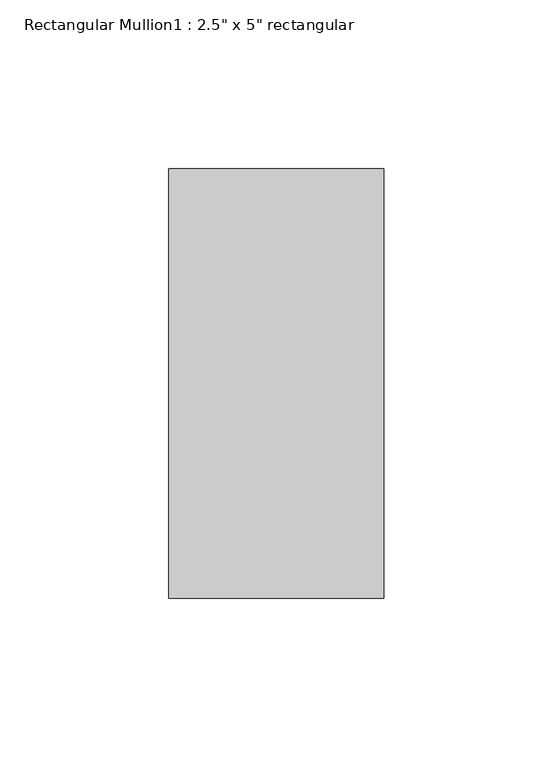
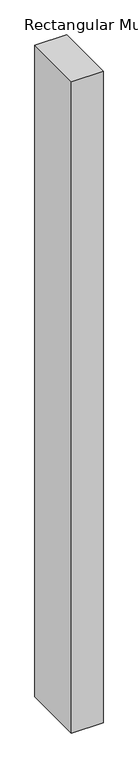
"""IFC4 building model written with IfcOpenShell, lengths in millimetres: member geometry."""

from ifc_helpers import new_model, si_unit, frame, origin, place, context, project, spatial, polyline, outline, extrude, source, transform, mapped, element, save


def member_8caa64b4(model_context):
    return source(origin(), model_context, "Body", "SweptSolid", [
        extrude(outline(polyline([(31.75, 63.5), (31.75, -63.5), (-31.75, -63.5), (-31.75, 63.5), (31.75, 63.5)])), frame((0.0, 0.0, -1383.5673076), z_axis=(0.0, 0.0, 1.0), x_axis=(1.0, 0.0, 0.0)), (0.0, 0.0, 1.0), 1383.5673076),
    ])


if __name__ == "__main__":
    model = new_model("IFC4")
    model_context = context("Model", 3, world=origin())
    ifc_project = project(units=[si_unit("LENGTHUNIT", "METRE", prefix="MILLI")], contexts=[model_context])
    site = spatial("IfcSite", under=ifc_project)
    building = spatial("IfcBuilding", under=site)
    placement = place(None, origin())
    member_shape = member_8caa64b4(model_context)
    element("IfcMember", 1, ObjectType="Rectangular Mullion1 : 2.5\" x 5\" rectangular", at=placement, inside=building, context=model_context, shape_type="MappedRepresentation", body=[
        mapped(member_shape, transform((0.0, 0.0, 0.0), x_axis=(1.0, 0.0, 0.0), y_axis=(0.0, 1.0, 0.0), z_axis=(0.0, 0.0, 1.0))),
    ])
    save(model, "model.ifc")

# Revit data of these elements
# Type "Rectangular Mullion1 : 2.5\" x 5\" rectangular"
#   built-in parameter 1007304 = 0.416667 (stored number, unit not read)
#   built-in parameter 1007301 = 0.104167 (stored number, unit not read)
#   built-in parameter 1007300 = 0.104167 (stored number, unit not read)
# Element 1 (IfcMember, "Rectangular Mullion1 : 2.5\" x 5\" rectangular")
#   Materials on its faces: "support-frame"
# Materials
#   "support-frame": class "Unassigned", colour RGB 233 233 233, transparency 0, Cost = 0
